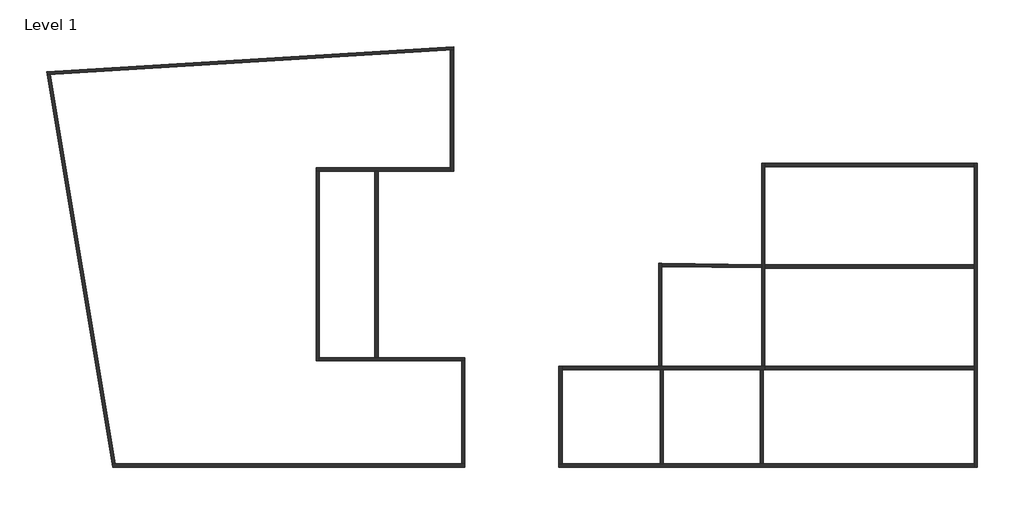
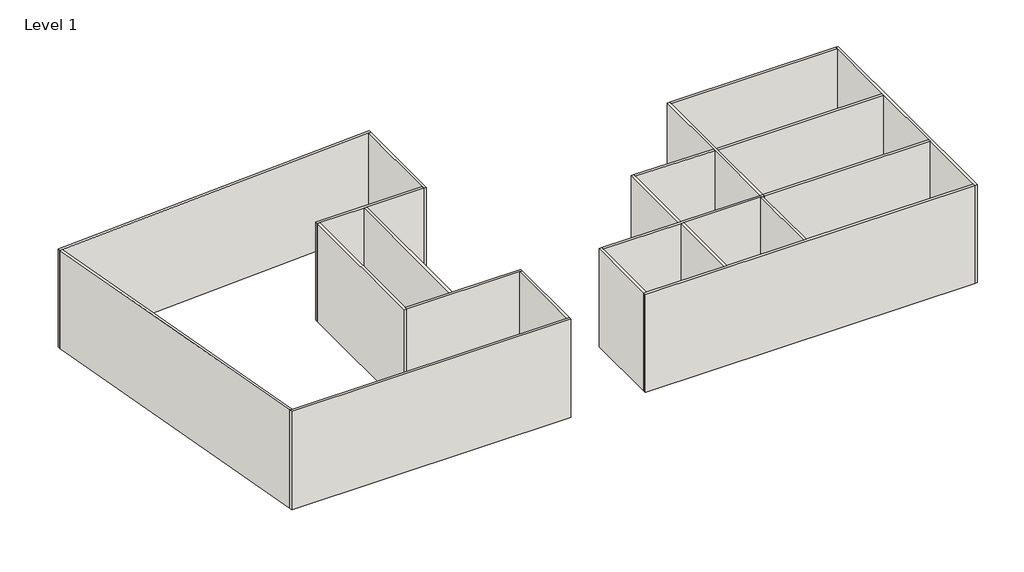
# One storey: 21 walls.
"""IFC4 building model written with IfcOpenShell, lengths in millimetres."""

from ifc_helpers import new_model, si_unit, origin, origin_with_axes, place, context, project, spatial, polyline, outline, extrude, faceted_brep, element, save

model = new_model("IFC4")

# Units and contexts
model_context = context("Model", 3, world=origin())
ifc_project = project(units=[si_unit("LENGTHUNIT", "METRE", prefix="MILLI")], contexts=[model_context])

# Site, building, storey
site = spatial("IfcSite", under=ifc_project)
building = spatial("IfcBuilding", under=site)
storey = spatial("IfcBuildingStorey", under=building, Name="Level 1", Elevation=0.0)

# Walls
placement = place(None, origin())
element("IfcWall", 1, ObjectType="Generic - 200mm", at=placement, inside=storey, context=model_context, shape_type="Brep", body=[
    faceted_brep([(30385.5457783, -10355.6072751, 0.0), (30385.5457783, 8204.197487, 0.0), (30385.5457783, 8204.197487, 8000.0), (30385.5457783, -10355.6072751, 8000.0), (30185.5457783, -10355.6072751, 0.0), (30185.5457783, -10355.6072751, 8000.0), (30185.5457783, -10155.6072751, 8000.0), (30185.5457783, -4395.802513, 8000.0), (30185.5457783, -4195.802513, 8000.0), (30185.5457783, 1804.197487, 8000.0), (30185.5457783, 2004.197487, 8000.0), (30185.5457783, 8004.197487, 8000.0), (30185.5457783, 8204.197487, 8000.0), (30185.5457783, 8204.197487, 0.0), (30185.5457783, 8004.197487, 0.0), (30185.5457783, 2004.197487, 0.0), (30185.5457783, 1804.197487, 0.0), (30185.5457783, -4195.802513, 0.0), (30185.5457783, -4395.802513, 0.0), (30185.5457783, -10155.6072751, 0.0)], [[[0, 1, 2, 3]], [[4, 5, 6, 7, 8, 9, 10, 11, 12, 13, 14, 15, 16, 17, 18, 19]], [[1, 0, 4, 19, 18, 17, 16, 15, 14, 13]], [[3, 2, 12, 11, 10, 9, 8, 7, 6, 5]], [[0, 3, 5, 4]], [[2, 1, 13, 12]]]),
])
element("IfcWall", 2, ObjectType="Generic - 200mm", at=placement, inside=storey, context=model_context, shape_type="Brep", body=[
    faceted_brep([(4799.1027843, -10355.6072751, 0.0), (30185.5457783, -10355.6072751, 0.0), (30185.5457783, -10355.6072751, 8000.0), (4799.1027843, -10355.6072751, 8000.0), (4799.1027843, -10155.6072751, 0.0), (4799.1027843, -10155.6072751, 8000.0), (4999.1027843, -10155.6072751, 8000.0), (10999.1027843, -10155.6072751, 8000.0), (11199.1027843, -10155.6072751, 8000.0), (17099.1027843, -10155.6072751, 8000.0), (17299.1027843, -10155.6072751, 8000.0), (30185.5457783, -10155.6072751, 8000.0), (30185.5457783, -10155.6072751, 0.0), (17299.1027843, -10155.6072751, 0.0), (17099.1027843, -10155.6072751, 0.0), (11199.1027843, -10155.6072751, 0.0), (10999.1027843, -10155.6072751, 0.0), (4999.1027843, -10155.6072751, 0.0)], [[[0, 1, 2, 3]], [[4, 5, 6, 7, 8, 9, 10, 11, 12, 13, 14, 15, 16, 17]], [[1, 0, 4, 17, 16, 15, 14, 13, 12]], [[3, 2, 11, 10, 9, 8, 7, 6, 5]], [[0, 3, 5, 4]], [[2, 1, 12, 11]]]),
])
element("IfcWall", 3, ObjectType="Generic - 200mm", at=placement, inside=storey, context=model_context, shape_type="Brep", body=[
    faceted_brep([(4799.1027843, -4195.802513, 0.0), (4799.1027843, -10155.6072751, 0.0), (4799.1027843, -10155.6072751, 8000.0), (4799.1027843, -4195.802513, 8000.0), (4999.1027843, -4195.802513, 0.0), (4999.1027843, -4195.802513, 8000.0), (4999.1027843, -4395.802513, 8000.0), (4999.1027843, -10155.6072751, 8000.0), (4999.1027843, -10155.6072751, 0.0), (4999.1027843, -4395.802513, 0.0)], [[[0, 1, 2, 3]], [[4, 5, 6, 7, 8, 9]], [[1, 0, 4, 9, 8]], [[3, 2, 7, 6, 5]], [[2, 1, 8, 7]], [[0, 3, 5, 4]]]),
])
element("IfcWall", 4, ObjectType="Generic - 200mm", at=placement, inside=storey, context=model_context, shape_type="Brep", body=[
    faceted_brep([(-26469.0109858, 13619.7899233, 0.0), (-26268.3017318, 13632.1480627, 0.0), (-1831.0745135, 15136.8054448, 0.0), (-1631.0745135, 15149.1199137, 0.0), (-1631.0745135, 15149.1199137, 8000.0), (-1831.0745135, 15136.8054448, 8000.0), (-26268.3017318, 13632.1480627, 8000.0), (-26469.0109858, 13619.7899233, 8000.0), (-26502.1654959, 13818.1272791, 0.0), (-26502.1654959, 13818.1272791, 8000.0), (-1631.0745135, 15349.4986705, 8000.0), (-1631.0745135, 15349.4986705, 0.0)], [[[0, 1, 2, 3, 4, 5, 6, 7]], [[8, 9, 10, 11]], [[3, 2, 1, 0, 8, 11]], [[7, 6, 5, 4, 10, 9]], [[0, 7, 9, 8]], [[4, 3, 11, 10]]]),
])
element("IfcWall", 5, ObjectType="Generic - 200mm", at=placement, inside=storey, context=model_context, shape_type="SweptSolid", body=[
    extrude(outline(polyline([(-26268.3017318, 13632.1480627), (-22291.888055, -10155.6072751), (-22494.6631228, -10155.6072751), (-26469.0109858, 13619.7899233), (-26268.3017318, 13632.1480627)])), origin_with_axes(), (0.0, 0.0, 1.0), 8000.0),
])
element("IfcWall", 6, ObjectType="Generic - 200mm", at=placement, inside=storey, context=model_context, shape_type="Brep", body=[
    faceted_brep([(-942.4446045, -10155.6072751, 0.0), (-1142.4446045, -10155.6072751, 0.0), (-22291.888055, -10155.6072751, 0.0), (-22494.6631228, -10155.6072751, 0.0), (-22494.6631228, -10155.6072751, 8000.0), (-22291.888055, -10155.6072751, 8000.0), (-1142.4446045, -10155.6072751, 8000.0), (-942.4446045, -10155.6072751, 8000.0), (-942.4446045, -10355.6072751, 0.0), (-942.4446045, -10355.6072751, 8000.0), (-22461.2306814, -10355.6072751, 8000.0), (-22461.2306814, -10355.6072751, 0.0)], [[[0, 1, 2, 3, 4, 5, 6, 7]], [[8, 9, 10, 11]], [[3, 2, 1, 0, 8, 11]], [[7, 6, 5, 4, 10, 9]], [[4, 3, 11, 10]], [[0, 7, 9, 8]]]),
])
element("IfcWall", 7, ObjectType="Generic - 200mm", at=placement, inside=storey, context=model_context, shape_type="Brep", body=[
    faceted_brep([(4999.1027843, -4395.802513, 0.0), (10999.1027843, -4395.802513, 0.0), (11199.1027843, -4395.802513, 0.0), (17099.1027843, -4395.802513, 0.0), (17299.1027843, -4395.802513, 0.0), (17399.1027843, -4395.802513, 0.0), (17399.1027843, -4395.802513, 8000.0), (17299.1027843, -4395.802513, 8000.0), (17099.1027843, -4395.802513, 8000.0), (11199.1027843, -4395.802513, 8000.0), (10999.1027843, -4395.802513, 8000.0), (4999.1027843, -4395.802513, 8000.0), (4999.1027843, -4195.802513, 0.0), (4999.1027843, -4195.802513, 8000.0), (10899.1027843, -4195.802513, 8000.0), (11099.1027843, -4195.802513, 8000.0), (17199.1027843, -4195.802513, 8000.0), (17399.1027843, -4195.802513, 8000.0), (17399.1027843, -4195.802513, 0.0), (17199.1027843, -4195.802513, 0.0), (11099.1027843, -4195.802513, 0.0), (10899.1027843, -4195.802513, 0.0)], [[[0, 1, 2, 3, 4, 5, 6, 7, 8, 9, 10, 11]], [[12, 13, 14, 15, 16, 17, 18, 19, 20, 21]], [[5, 4, 3, 2, 1, 0, 12, 21, 20, 19, 18]], [[11, 10, 9, 8, 7, 6, 17, 16, 15, 14, 13]], [[0, 11, 13, 12]], [[6, 5, 18, 17]]]),
])
element("IfcWall", 8, ObjectType="Generic - 200mm", at=placement, inside=storey, context=model_context, shape_type="Brep", body=[
    faceted_brep([(17399.1027843, -4195.802513, 0.0), (17399.1027843, 1804.197487, 0.0), (17399.1027843, 2004.197487, 0.0), (17399.1027843, 8004.197487, 0.0), (17399.1027843, 8204.197487, 0.0), (17399.1027843, 8204.197487, 8000.0), (17399.1027843, 8004.197487, 8000.0), (17399.1027843, 2004.197487, 8000.0), (17399.1027843, 1804.197487, 8000.0), (17399.1027843, -4195.802513, 8000.0), (17199.1027843, -4195.802513, 0.0), (17199.1027843, -4195.802513, 8000.0), (17199.1027843, 1821.0486348, 8000.0), (17199.1027843, 2021.0665631, 8000.0), (17199.1027843, 8204.197487, 8000.0), (17199.1027843, 8204.197487, 0.0), (17199.1027843, 2021.0665631, 0.0), (17199.1027843, 1821.0486348, 0.0)], [[[0, 1, 2, 3, 4, 5, 6, 7, 8, 9]], [[10, 11, 12, 13, 14, 15, 16, 17]], [[4, 3, 2, 1, 0, 10, 17, 16, 15]], [[9, 8, 7, 6, 5, 14, 13, 12, 11]], [[0, 9, 11, 10]], [[5, 4, 15, 14]]]),
])
element("IfcWall", 9, ObjectType="Generic - 200mm", at=placement, inside=storey, context=model_context, shape_type="SweptSolid", body=[
    extrude(outline(polyline([(30185.5457783, 8004.197487), (17399.1027843, 8004.197487), (17399.1027843, 8204.197487), (30185.5457783, 8204.197487), (30185.5457783, 8004.197487)])), origin_with_axes(), (0.0, 0.0, 1.0), 8000.0),
])
element("IfcWall", 10, ObjectType="Generic - 200mm", at=placement, inside=storey, context=model_context, shape_type="Brep", body=[
    faceted_brep([(-1831.0745135, 15136.8054448, 0.0), (-1831.0745135, 7936.8054448, 0.0), (-1831.0745135, 7736.8054448, 0.0), (-1831.0745135, 7736.8054448, 8000.0), (-1831.0745135, 7936.8054448, 8000.0), (-1831.0745135, 15136.8054448, 8000.0), (-1631.0745135, 15149.1199137, 0.0), (-1631.0745135, 15149.1199137, 8000.0), (-1631.0745135, 7736.8054448, 8000.0), (-1631.0745135, 7736.8054448, 0.0)], [[[0, 1, 2, 3, 4, 5]], [[6, 7, 8, 9]], [[2, 1, 0, 6, 9]], [[5, 4, 3, 8, 7]], [[0, 5, 7, 6]], [[3, 2, 9, 8]]]),
])
element("IfcWall", 11, ObjectType="Generic - 200mm", at=placement, inside=storey, context=model_context, shape_type="Brep", body=[
    faceted_brep([(-1831.0745135, 7936.8054448, 0.0), (-10031.0745135, 7936.8054448, 0.0), (-10031.0745135, 7936.8054448, 8000.0), (-1831.0745135, 7936.8054448, 8000.0), (-1831.0745135, 7736.8054448, 0.0), (-1831.0745135, 7736.8054448, 8000.0), (-6231.0745135, 7736.8054448, 8000.0), (-6431.0745135, 7736.8054448, 8000.0), (-9831.0745135, 7736.8054448, 8000.0), (-10031.0745135, 7736.8054448, 8000.0), (-10031.0745135, 7736.8054448, 0.0), (-9831.0745135, 7736.8054448, 0.0), (-6431.0745135, 7736.8054448, 0.0), (-6231.0745135, 7736.8054448, 0.0)], [[[0, 1, 2, 3]], [[4, 5, 6, 7, 8, 9, 10, 11, 12, 13]], [[1, 0, 4, 13, 12, 11, 10]], [[3, 2, 9, 8, 7, 6, 5]], [[0, 3, 5, 4]], [[2, 1, 10, 9]]]),
])
element("IfcWall", 12, ObjectType="Generic - 200mm", at=placement, inside=storey, context=model_context, shape_type="Brep", body=[
    faceted_brep([(-10031.0745135, 7736.8054448, 0.0), (-10031.0745135, -3863.1945552, 0.0), (-10031.0745135, -3863.1945552, 8000.0), (-10031.0745135, 7736.8054448, 8000.0), (-9831.0745135, 7736.8054448, 0.0), (-9831.0745135, 7736.8054448, 8000.0), (-9831.0745135, -3663.1945552, 8000.0), (-9831.0745135, -3863.1945552, 8000.0), (-9831.0745135, -3863.1945552, 0.0), (-9831.0745135, -3663.1945552, 0.0)], [[[0, 1, 2, 3]], [[4, 5, 6, 7, 8, 9]], [[1, 0, 4, 9, 8]], [[3, 2, 7, 6, 5]], [[0, 3, 5, 4]], [[2, 1, 8, 7]]]),
])
element("IfcWall", 13, ObjectType="Generic - 200mm", at=placement, inside=storey, context=model_context, shape_type="Brep", body=[
    faceted_brep([(-9831.0745135, -3863.1945552, 0.0), (-1142.4446045, -3863.1945552, 0.0), (-942.4446045, -3863.1945552, 0.0), (-942.4446045, -3863.1945552, 8000.0), (-1142.4446045, -3863.1945552, 8000.0), (-9831.0745135, -3863.1945552, 8000.0), (-9831.0745135, -3663.1945552, 0.0), (-9831.0745135, -3663.1945552, 8000.0), (-6431.0745135, -3663.1945552, 8000.0), (-6231.0745135, -3663.1945552, 8000.0), (-942.4446045, -3663.1945552, 8000.0), (-942.4446045, -3663.1945552, 0.0), (-6231.0745135, -3663.1945552, 0.0), (-6431.0745135, -3663.1945552, 0.0)], [[[0, 1, 2, 3, 4, 5]], [[6, 7, 8, 9, 10, 11, 12, 13]], [[2, 1, 0, 6, 13, 12, 11]], [[5, 4, 3, 10, 9, 8, 7]], [[0, 5, 7, 6]], [[3, 2, 11, 10]]]),
])
element("IfcWall", 14, ObjectType="Generic - 200mm", at=placement, inside=storey, context=model_context, shape_type="SweptSolid", body=[
    extrude(outline(polyline([(-1142.4446045, -10155.6072751), (-1142.4446045, -3863.1945552), (-942.4446045, -3863.1945552), (-942.4446045, -10155.6072751), (-1142.4446045, -10155.6072751)])), origin_with_axes(), (0.0, 0.0, 1.0), 8000.0),
])
element("IfcWall", 15, ObjectType="Generic - 200mm", at=placement, inside=storey, context=model_context, shape_type="SweptSolid", body=[
    extrude(outline(polyline([(30185.5457783, 1804.197487), (17399.1027843, 1804.197487), (17399.1027843, 2004.197487), (30185.5457783, 2004.197487), (30185.5457783, 1804.197487)])), origin_with_axes(), (0.0, 0.0, 1.0), 8000.0),
])
element("IfcWall", 16, ObjectType="Generic - 200mm", at=placement, inside=storey, context=model_context, shape_type="SweptSolid", body=[
    extrude(outline(polyline([(30185.5457783, -4395.802513), (17399.1027843, -4395.802513), (17399.1027843, -4195.802513), (30185.5457783, -4195.802513), (30185.5457783, -4395.802513)])), origin_with_axes(), (0.0, 0.0, 1.0), 8000.0),
])
element("IfcWall", 17, ObjectType="Generic - 200mm", at=placement, inside=storey, context=model_context, shape_type="SweptSolid", body=[
    extrude(outline(polyline([(10999.1027843, -10155.6072751), (10999.1027843, -4395.802513), (11199.1027843, -4395.802513), (11199.1027843, -10155.6072751), (10999.1027843, -10155.6072751)])), origin_with_axes(), (0.0, 0.0, 1.0), 8000.0),
])
element("IfcWall", 18, ObjectType="Generic - 200mm", at=placement, inside=storey, context=model_context, shape_type="SweptSolid", body=[
    extrude(outline(polyline([(17099.1027843, -10155.6072751), (17099.1027843, -4395.802513), (17299.1027843, -4395.802513), (17299.1027843, -10155.6072751), (17099.1027843, -10155.6072751)])), origin_with_axes(), (0.0, 0.0, 1.0), 8000.0),
])
element("IfcWall", 19, ObjectType="Generic - 200mm", at=placement, inside=storey, context=model_context, shape_type="Brep", body=[
    faceted_brep([(11099.1027843, -4195.802513, 0.0), (11099.1027843, 1902.7272763, 0.0), (11099.1027843, 2102.7452045, 0.0), (11099.1027843, 2102.7452045, 8000.0), (11099.1027843, 1902.7272763, 8000.0), (11099.1027843, -4195.802513, 8000.0), (10899.1027843, -4195.802513, 0.0), (10899.1027843, -4195.802513, 8000.0), (10899.1027843, 2105.4231928, 8000.0), (10899.1027843, 2105.4231928, 0.0)], [[[0, 1, 2, 3, 4, 5]], [[6, 7, 8, 9]], [[2, 1, 0, 6, 9]], [[5, 4, 3, 8, 7]], [[0, 5, 7, 6]], [[3, 2, 9, 8]]]),
])
element("IfcWall", 20, ObjectType="Generic - 200mm", at=placement, inside=storey, context=model_context, shape_type="SweptSolid", body=[
    extrude(outline(polyline([(17199.1027843, 1821.0486348), (11099.1027843, 1902.7272763), (11099.1027843, 2102.7452045), (17199.1027843, 2021.0665631), (17199.1027843, 1821.0486348)])), origin_with_axes(), (0.0, 0.0, 1.0), 8000.0),
])
element("IfcWall", 21, ObjectType="Generic - 200mm", at=placement, inside=storey, context=model_context, shape_type="SweptSolid", body=[
    extrude(outline(polyline([(-6431.0745135, -3663.1945552), (-6431.0745135, 7736.8054448), (-6231.0745135, 7736.8054448), (-6231.0745135, -3663.1945552), (-6431.0745135, -3663.1945552)])), origin_with_axes(), (0.0, 0.0, 1.0), 8000.0),
])

save(model, "model.ifc")

# Revit data of these elements
# Project information
#   Project Issue Date = "Issue Date"
#   Project Status = "Project Status"
#   Client Name = "Owner"
#   Project Address = "Enter address here"
#   Project Name = "Project Name"
#   Project Number = "0001"
# Type "Generic - 200mm"
#   Layers, outside or top first: 20 cm no material (function 1)
# Elements 1, 2, 3, 4, 5, 6, 7, 8, 9, 10, 11, 12, 13, 14, 15, 16, 17, 18, 19, 20, 21 (IfcWall, "Generic - 200mm")
#   Top Offset = 0 cm
#   Base Offset = 0 cm
#   Unconnected Height = 800 cm
#   wall height = 800 cm
#   Phase Created = New Construction
#   Base Constraint = Level 1
#   Materials on its faces: "Default Wall"
# Materials
#   "Default Wall": class "Miscellaneous", colour RGB 128 128 128, transparency 0, Cost = 0
# Room, not placed, phase "New Construction", upper offset 0 cm, lower offset 0 cm
#   Number = "5"
#   Name = "Room"
# Room, not placed, phase "New Construction", upper offset 0 cm, lower offset 0 cm
#   Number = "6"
#   Name = "Room"
# Area, not placed, upper offset 0 cm, lower offset 0 cm
#   Number = "2"
#   Name = "Area"
# Room, not placed, phase "New Construction", upper offset 0 cm, lower offset 0 cm
#   Number = "1"
#   Name = "Room"
# Area, not placed, upper offset 0 cm, lower offset 0 cm
#   Number = "3"
#   Name = "Area"
# Room at (16426.208, -6054.156) mm, phase "New Construction", upper level "Level 1", upper offset 243.84 cm, lower offset 0 cm
#   Number = "7"
#   Name = "Room"
# Room at (-17959.319, 362.594) mm, phase "New Construction", upper level "Level 1", upper offset 243.84 cm, lower offset 0 cm
#   Number = "8"
#   Name = "Room"
# Room, not placed, phase "New Construction", upper offset 0 cm, lower offset 0 cm
#   Number = "2"
#   Name = "Room"
# Room, not placed, phase "New Construction", upper offset 0 cm, lower offset 0 cm
#   Number = "3"
#   Name = "Room"
# Room, not placed, phase "New Construction", upper offset 0 cm, lower offset 0 cm
#   Number = "4"
#   Name = "Room"
# Area, not placed, upper offset 0 cm, lower offset 0 cm
#   Number = "1"
#   Name = "Area"
